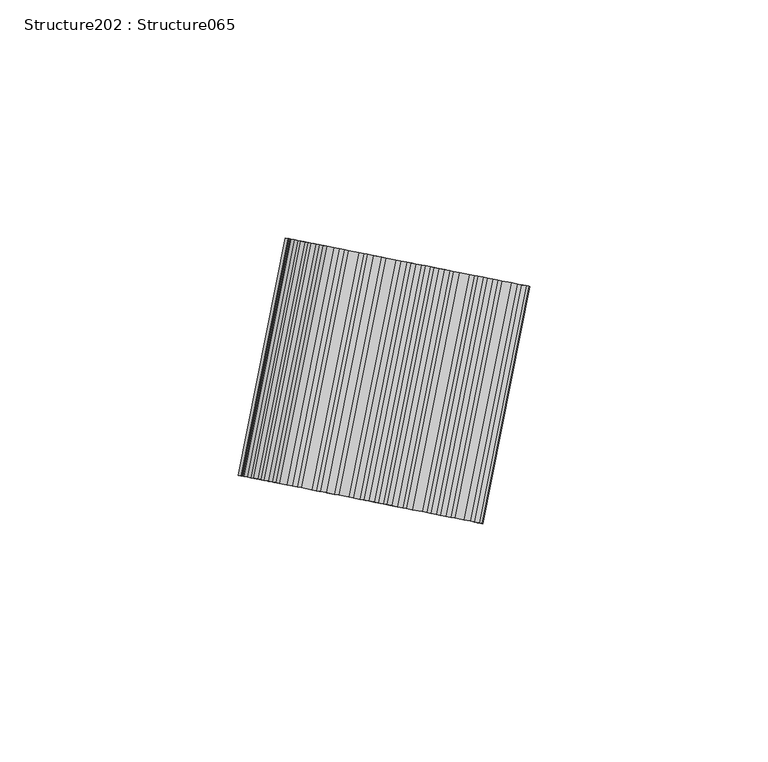
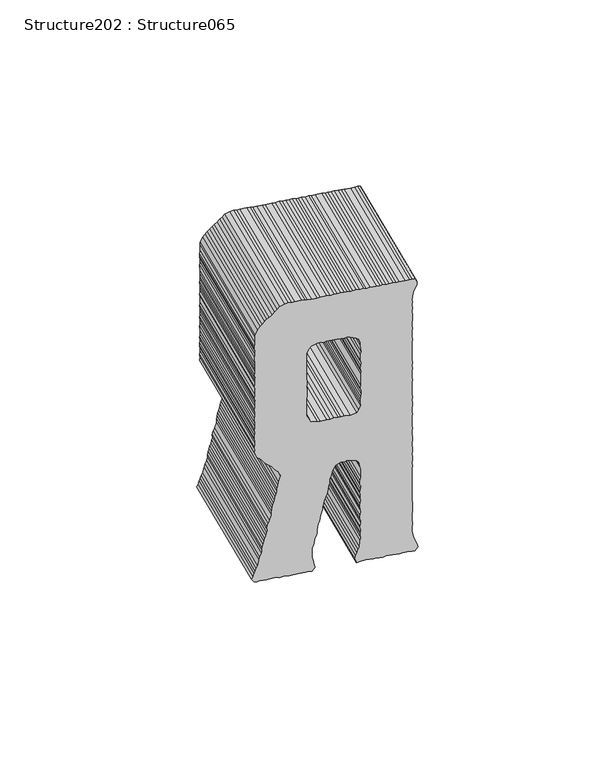
"""IFC4 building model written with IfcOpenShell, lengths in millimetres: proxy geometry, Structure202 : Structure065."""

from ifc_helpers import new_model, si_unit, frame, origin, place, context, project, spatial, polyline, outline, extrude, source, transform, mapped, element, save


def structure202_structure065_2f925049(model_context):
    return source(origin(), model_context, "Body", "SweptSolid", [
        extrude(outline(polyline([(0.7871188, 0.0), (1.9467099, -0.1934423), (2.8611126, -0.2132328), (4.1212942, -0.5562052), (5.0176609, -0.7057366), (5.8930671, -0.9830781), (7.2176514, -0.9399881), (7.9671776, -1.1977733), (10.1456225, -1.5611803), (11.3169321, -1.6238278), (12.3202067, -1.9239432), (13.220785, -2.0741771), (14.2235918, -2.3727715), (15.4221794, -2.3086628), (16.5332978, -2.7580753), (17.4474664, -2.7792697), (18.628954, -2.8436151), (20.3760226, -3.3991165), (21.6573988, -3.612875), (22.5973246, -3.5056165), (23.7042315, -3.9543264), (24.6497726, -3.8480047), (25.7998876, -4.0398662), (26.5259967, -4.4250517), (27.5508168, -4.5960116), (28.8750501, -4.5528631), (29.8605229, -4.9813155), (30.8000977, -4.8739984), (32.5717532, -6.0908565), (32.9377317, -7.0757454), (33.5964553, -7.843249), (34.5198072, -8.6548979), (35.1339188, -9.6790158), (36.0291146, -11.4098042), (36.929166, -12.3503157), (37.5875383, -13.1199252), (37.9967252, -13.8458014), (39.5794443, -14.6361387), (41.715559, -14.4661751), (43.0356389, -14.4241374), (43.9753304, -14.3182827), (45.1310609, -14.5110811), (46.0922399, -14.2742577), (47.0321656, -14.1669992), (48.2092074, -14.2320458), (49.1644782, -13.9960405), (50.1096681, -13.8918246), (51.1536357, -13.9328682), (52.2245298, -13.8492615), (53.5020455, -14.062376), (55.3872199, -13.8483862), (56.4950633, -13.5065261), (57.6901412, -13.441832), (58.8221031, -13.7641363), (59.6518448, -13.5086332), (60.8291209, -13.5722761), (61.6842107, -13.1864482), (62.8570992, -13.2526058), (63.8005346, -13.1459327), (64.9935066, -13.0808873), (65.8902243, -13.2304772), (66.9632246, -13.1450574), (68.1987025, -12.8252108), (69.3917916, -12.7594634), (71.3806564, -12.6980459), (72.2372083, -12.3142657), (73.3027212, -12.2283183), (74.1379616, -11.9722895), (75.3345602, -11.9092919), (76.060085, -11.5022109), (76.9541114, -12.442078), (76.9148807, -13.4881518), (76.654873, -14.2358643), (76.6153496, -15.2836929), (76.4231953, -16.4355627), (76.1203305, -17.4401822), (75.7994879, -19.3634749), (75.9089108, -20.303401), (75.4361395, -21.5415689), (75.3958554, -23.3789145), (75.0550475, -24.636932), (74.5630694, -27.5860978), (74.5408216, -28.5044193), (74.1318675, -29.3600344), (74.2202717, -30.4259572), (72.7677599, -31.2380719), (71.9348595, -30.7059292), (70.9319944, -30.4055214), (69.81877, -29.9557576), (69.092661, -29.5705721), (67.0454774, -29.2290621), (65.8897469, -29.0362638), (64.9073151, -29.4004879), (63.9889933, -29.3804043), (62.8179181, -29.3141885), (61.8295198, -29.6774173), (60.6364307, -29.7431646), (59.5910013, -29.697909), (58.5414768, -29.6555776), (57.4974509, -29.6127205), (56.5096379, -29.9746039), (55.3383286, -29.909792), (54.2921966, -29.868748), (53.1997568, -30.0815101), (52.2660902, -30.1880091), (51.3634061, -30.0374239), (50.1703755, -30.1028203), (49.1034001, -30.1888844), (48.011253, -30.3998918), (47.2025297, -30.5315625), (45.9829235, -30.7216679), (45.0646604, -30.699069), (43.8681202, -30.76388), (42.9281945, -30.8711385), (41.6450635, -30.6570873), (40.8369841, -30.7848975), (39.744193, -30.9997654), (38.4199597, -31.0429139), (36.6021707, -31.6617043), (35.708143, -33.0918511), (35.4943845, -34.3732273), (35.1130015, -35.098167), (35.152289, -36.4239206), (35.3651098, -38.3031284), (36.0274012, -39.0730309), (37.5039731, -39.7125504), (38.6111139, -40.1620209), (41.55677, -40.6534136), (42.628074, -40.56735), (43.9094502, -40.7811085), (44.8909452, -41.2096188), (45.9402356, -41.2533541), (46.7273548, -41.2511897), (47.7284065, -41.5516557), (49.0153982, -41.7663509), (49.8872947, -42.043107), (51.0842445, -41.9780036), (52.1143292, -42.1498417), (52.8581229, -42.4073921), (53.8647903, -42.7066306), (55.1894917, -42.6628386), (56.2136099, -42.8336814), (57.0677044, -43.2409389), (57.964422, -43.3905288), (59.1613719, -43.3254254), (60.2702675, -43.7751886), (61.3142934, -43.8180457), (62.0853653, -43.9466754), (63.2180294, -44.2669326), (64.1538607, -44.1582695), (66.5064238, -44.2866665), (67.3413129, -44.0327435), (68.6659557, -43.9893025), (69.5168336, -43.6049364), (70.7154797, -43.5404768), (71.9110832, -44.2684001), (71.5698656, -45.5288744), (71.1417649, -46.5100771), (70.9918236, -47.4089005), (70.9678209, -48.3269293), (70.9073373, -49.5004036), (70.6044725, -50.5050232), (70.5864362, -51.4240472), (70.4152421, -52.4502714), (70.008687, -53.3023186), (69.96308, -54.3498537), (69.5997902, -56.5275967), (69.5604425, -57.5743723), (69.2792403, -58.4491346), (68.9155992, -60.6289832), (68.8979142, -61.5459015), (68.7482657, -62.4429702), (67.444349, -63.1492881), (66.3524357, -62.573937), (65.5024946, -62.1655689), (64.4335891, -61.46311), (63.7054328, -61.0772222), (61.7402195, -60.2227166), (60.7157503, -60.0518152), (58.6206793, -59.9649302), (57.7721999, -59.5607738), (56.4677578, -59.4723099), (55.5881396, -59.1964301), (54.5210475, -59.2810319), (51.5715307, -58.7889952), (50.5917903, -58.362942), (49.567321, -58.1920406), (48.2590183, -58.1029326), (46.3434468, -57.7833781), (45.336428, -57.4862454), (44.3137137, -57.3156368), (43.2682842, -57.2703812), (39.296404, -56.6077944), (38.2502721, -56.5667504), (37.243956, -56.2654062), (35.9388112, -56.1811538), (34.9164478, -56.0106037), (34.1666876, -55.752058), (33.1226615, -55.7113653), (31.8353188, -55.4966115), (30.8325124, -55.1958528), (29.9414101, -55.0471996), (29.0174143, -55.0265303), (27.8672993, -54.8346688), (27.0093439, -54.4289317), (25.8361629, -54.3623646), (24.7921367, -54.3216719), (23.6846447, -53.8743072), (22.8887519, -53.8706792), (21.8852429, -53.5741321), (20.5829065, -53.4860194), (19.5371255, -53.4450339), (18.8100804, -53.0611352), (17.5269493, -52.847084), (16.7185191, -52.9748356), (15.5589279, -52.7813933), (14.6894885, -52.5028827), (13.6437075, -52.4618973), (12.3780276, -52.1172862), (11.6335313, -51.8639473), (10.4624561, -51.7977316), (8.2783958, -51.4333879), (7.487767, -51.4349668), (6.3589637, -51.1131893), (5.4835572, -50.8380122), (4.3271248, -50.6450968), (3.3881352, -50.7510686), (2.259332, -50.4292911), (1.3356871, -50.4086803), (0.1004435, -49.9400042), (-0.9278864, -49.7684588), (-1.97121, -49.7235545), (-2.7160573, -49.4701571), (-3.7667512, -49.4240233), (-4.7685054, -49.1277689), (-6.0502326, -48.9139519), (-6.8639273, -49.0408253), (-8.1236408, -48.6972095), (-8.8741036, -48.4428754), (-9.896116, -48.2723838), (-10.9635591, -48.3569271), (-11.9698753, -48.0555828), (-13.2512515, -47.8418244), (-14.0439861, -47.843052), (-16.0908187, -47.5016005), (-17.2039263, -47.0532991), (-18.2692636, -47.1381936), (-19.3977159, -46.8164747), (-20.4498143, -46.7744354), (-21.3248692, -46.4949881), (-23.5459373, -46.3892486), (-24.6132635, -46.4752542), (-25.468002, -46.8589764), (-26.5569911, -47.0748392), (-27.732161, -47.0093833), (-28.6765316, -46.3237313), (-28.6309247, -45.276196), (-28.4816275, -44.3812332), (-28.1419891, -43.1194133), (-27.9467337, -41.1748095), (-27.6717907, -40.3008068), (-27.6265937, -39.2557283), (-27.4341467, -38.1021037), (-27.1585597, -37.2242404), (-27.0919341, -36.0507085), (-26.8380098, -35.3027026), (-26.7927543, -34.2572732), (-26.450366, -32.204825), (-26.1112545, -30.9461638), (-26.2363148, -30.1345752), (-25.7904704, -29.0232221), (-25.851655, -27.8287297), (-25.5527093, -26.8238171), (-25.2987265, -26.0754602), (-25.3808711, -25.0066135), (-25.1035297, -24.1312073), (-25.039127, -22.9580261), (-24.7405326, -21.9552192), (-24.7183429, -21.0350843), (-24.2514799, -19.7977346), (-24.205873, -18.7501994), (-23.7377804, -16.7183604), (-23.5672889, -15.696348), (-23.2893034, -14.0299623), (-23.0751936, -12.7464803), (-23.0728537, -11.9583088), (-23.0293525, -10.9104224), (-22.6659456, -8.7319775), (-22.3886627, -7.8569222), (-22.3451616, -6.8090358), (-21.89961, -5.6994376), (-21.1256712, -4.2496184), (-20.1054129, -3.6283696), (-19.3334628, -2.964616), (-18.3028511, -2.3461766), (-17.4942452, -1.4302533), (-16.8743997, -0.8717109), (-16.0026199, -0.3598857), (-15.0773951, 0.4096054), (-14.3584222, 0.8141722), (-13.2017553, 1.4119439), (-11.4074421, 1.902983), (-10.4894129, 1.8811446), (-8.4366139, 1.5386978), (-7.1375527, 1.4547389), (-6.3622691, 1.3254065), (-5.381008, 0.8976567), (-4.3582936, 0.7270481), (-3.2909673, 0.8130537), (-1.0241182, 0.1708428), (0.0, 0.0), (0.7871188, 0.0)]), holes=[polyline([(19.0863815, -31.6360536), (19.4317522, -30.3766329), (19.4281257, -29.5874661), (19.6422354, -28.3039841), (20.0937535, -27.1953812), (20.1372546, -26.1474947), (20.6074529, -24.116007), (20.4976205, -23.1763735), (20.5710904, -21.2136178), (19.7325749, -20.678374), (18.4726861, -19.546528), (17.5550665, -19.5243972), (16.2736902, -19.3106387), (15.5235202, -19.0545498), (14.3695447, -18.8620443), (13.4550837, -18.8404404), (12.4330713, -18.6699489), (11.1240659, -18.5850524), (9.0751274, -18.2432497), (8.0688113, -17.9419055), (7.1500799, -17.9221144), (6.2533623, -17.7725244), (5.1461629, -17.323405), (4.2494452, -17.173815), (3.0724619, -17.1084173), (2.1753932, -16.9587688), (1.1739318, -16.6607596), (-0.0030516, -16.5953619), (-0.8785164, -16.3183714), (-2.0342468, -16.1255731), (-2.9525684, -16.1033252), (-3.8224177, -15.8272715), (-5.4698907, -16.2122211), (-6.3692412, -16.8525574), (-7.4590496, -18.6454073), (-7.6303023, -19.6719823), (-7.501381, -20.4820506), (-7.9294821, -21.4654177), (-8.4641417, -24.6704375), (-8.5516106, -25.9710776), (-8.5489789, -26.7618821), (-8.9767287, -27.7431432), (-8.8910744, -28.8125754), (-8.5504439, -30.7149079), (-8.1628609, -31.5681261), (-6.711052, -32.3366251), (-5.8146853, -32.4861564), (-3.5476025, -33.1291278), (-2.6117711, -33.0204648), (-0.4336773, -33.3838131), (0.2930166, -33.7698177), (1.4700584, -33.8348644), (2.3884388, -33.8545969), (3.6233312, -34.3253789), (4.4136088, -34.3259058), (8.3875947, -34.9888439), (9.5628822, -35.0514335), (10.4169766, -35.458691), (11.4467103, -35.6304706), (12.6184877, -35.694639), (13.5372191, -35.7144301), (14.565198, -35.885917), (15.8210508, -36.2288888), (17.2098622, -35.8007893), (18.2192791, -35.3115638), (19.0465068, -33.4731068), (19.0863815, -31.6360536)])]), frame((-1973.7922668, 234860.1940729, 464.6145124), z_axis=(0.1946622229639412, 0.9808703374813295, 0.0), x_axis=(-0.16139789404123722, 0.032030811448979596, -0.9863694778920187)), (0.0, 0.0, 1.0), 50.8),
    ])


if __name__ == "__main__":
    model = new_model("IFC4")
    model_context = context("Model", 3, world=origin())
    ifc_project = project(units=[si_unit("LENGTHUNIT", "METRE", prefix="MILLI")], contexts=[model_context])
    site = spatial("IfcSite", under=ifc_project)
    building = spatial("IfcBuilding", under=site)
    placement = place(None, origin())
    structure202_structure065_shape = structure202_structure065_2f925049(model_context)
    element("IfcBuildingElementProxy", 1, Name="Structure202 : Structure065", ObjectType="Structure202 : Structure065", at=placement, inside=building, context=model_context, shape_type="MappedRepresentation", body=[
        mapped(structure202_structure065_shape, transform((0.0, 0.0, 0.0), x_axis=(1.0, 0.0, 0.0), y_axis=(0.0, 1.0, 0.0), z_axis=(0.0, 0.0, 1.0))),
    ])
    save(model, "model.ifc")

# Revit data of these elements
# Type "Structure202 : Structure065"
#   NameOverride = "Structure065"
# Element 1 (IfcBuildingElementProxy, "Structure202 : Structure065")
#   Materials on its faces: "BRUSHED ALUMINUM LETTERING"
# Materials
#   "BRUSHED ALUMINUM LETTERING": class "Unassigned", colour RGB 169 181 186, transparency 0, Cost = 0
